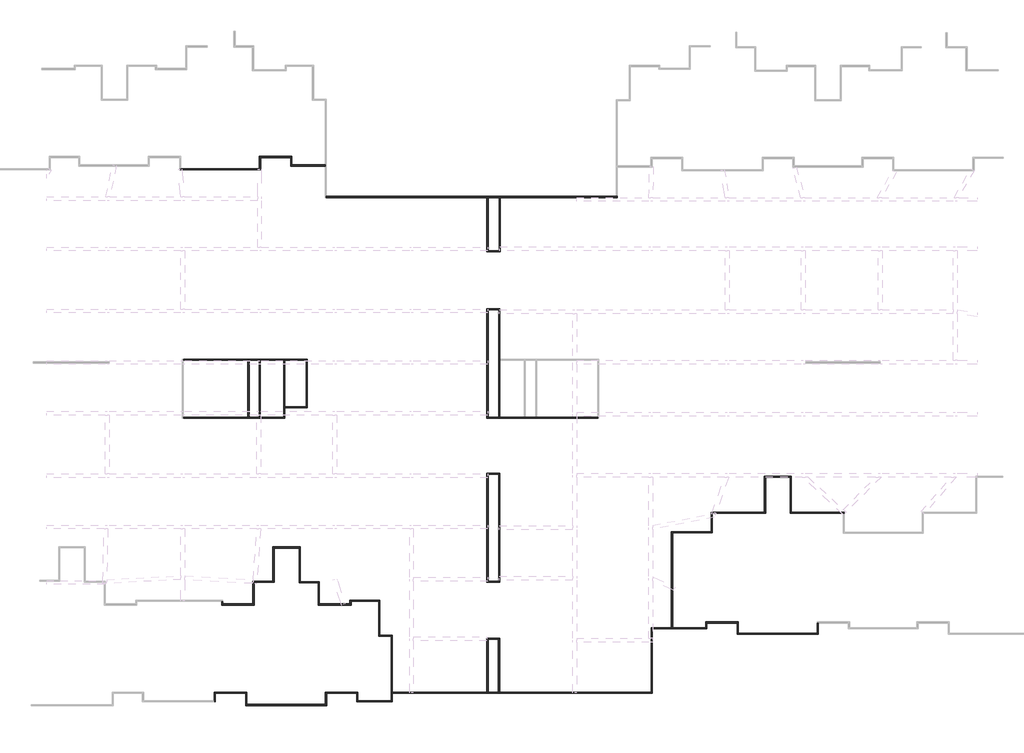
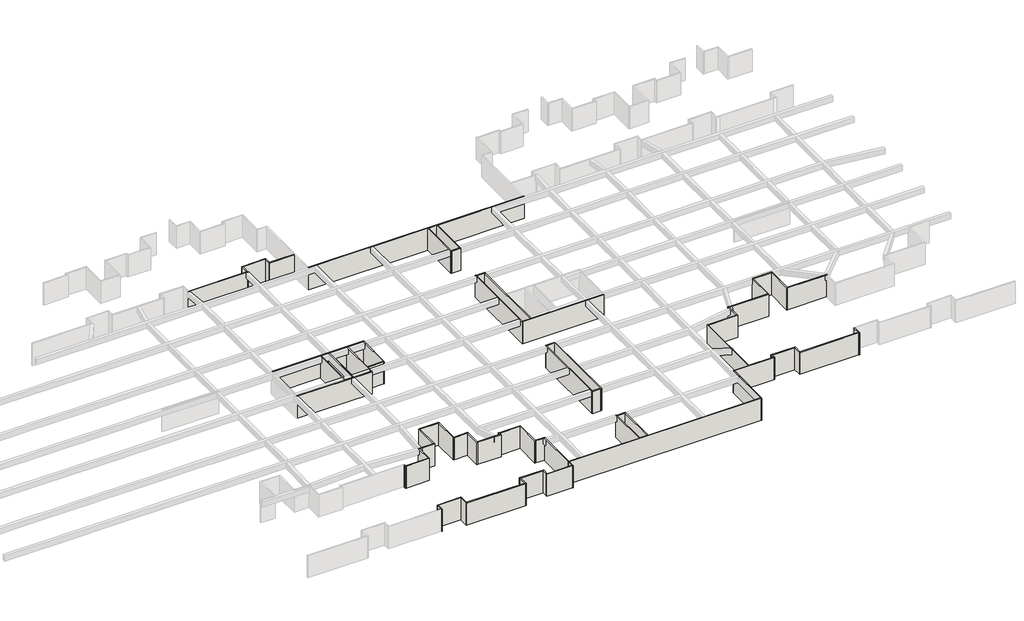
# One storey, part 6 of 16: 67 walls.
"""IFC4 building model written with IfcOpenShell, lengths in millimetres."""

from ifc_helpers import new_model, si_unit, origin, origin_with_axes, place, context, project, spatial, polyline, outline, extrude, faceted_brep, element, save

model = new_model("IFC4")

# Units and contexts
model_context = context("Model", 3, world=origin())
ifc_project = project(units=[si_unit("LENGTHUNIT", "METRE", prefix="MILLI")], contexts=[model_context])

# Site, building, storey
site = spatial("IfcSite", under=ifc_project)
building = spatial("IfcBuilding", under=site)
storey = spatial("IfcBuildingStorey", under=building, Name="户型图", Elevation=0.0)

# Walls
placement = place(None, origin())
element("IfcWall", 1, ObjectType="所有墙体", at=placement, inside=storey, context=model_context, shape_type="Brep", body=[
    faceted_brep([(396205.7298502, -128941.8026441, 0.0), (392717.9162298, -128941.8026441, 0.0), (392597.9162298, -128941.8026441, 0.0), (392597.9162298, -128941.8026441, 3300.0), (392717.9162298, -128941.8026441, 3300.0), (396205.7298502, -128941.8026441, 3300.0), (396205.7298502, -129061.8026441, 0.0), (396205.7298502, -129061.8026441, 3300.0), (392597.9162298, -129061.8026441, 3300.0), (392597.9162298, -129061.8026441, 0.0)], [[[0, 1, 2, 3, 4, 5]], [[6, 7, 8, 9]], [[2, 1, 0, 6, 9]], [[5, 4, 3, 8, 7]], [[0, 5, 7, 6]], [[3, 2, 9, 8]]]),
])
element("IfcWall", 2, ObjectType="所有墙体", at=placement, inside=storey, context=model_context, shape_type="Brep", body=[
    faceted_brep([(392717.9162298, -128941.8026441, 0.0), (392717.9162298, -128039.1416737, 0.0), (392717.9162298, -128039.1416737, 3300.0), (392717.9162298, -128941.8026441, 3300.0), (392597.9162298, -128941.8026441, 0.0), (392597.9162298, -128941.8026441, 3300.0), (392597.9162298, -128159.1416737, 3300.0), (392597.9162298, -128039.1416737, 3300.0), (392597.9162298, -128039.1416737, 0.0), (392597.9162298, -128159.1416737, 0.0)], [[[0, 1, 2, 3]], [[4, 5, 6, 7, 8, 9]], [[1, 0, 4, 9, 8]], [[3, 2, 7, 6, 5]], [[0, 3, 5, 4]], [[2, 1, 8, 7]]]),
])
element("IfcWall", 3, ObjectType="所有墙体", at=placement, inside=storey, context=model_context, shape_type="Brep", body=[
    faceted_brep([(392597.9162298, -128039.1416737, 0.0), (389297.1677555, -128039.1416737, 0.0), (389297.1677555, -128039.1416737, 3300.0), (392597.9162298, -128039.1416737, 3300.0), (392597.9162298, -128159.1416737, 0.0), (392597.9162298, -128159.1416737, 3300.0), (389417.1677555, -128159.1416737, 3300.0), (389297.1677555, -128159.1416737, 3300.0), (389297.1677555, -128159.1416737, 0.0), (389417.1677555, -128159.1416737, 0.0)], [[[0, 1, 2, 3]], [[4, 5, 6, 7, 8, 9]], [[1, 0, 4, 9, 8]], [[3, 2, 7, 6, 5]], [[0, 3, 5, 4]], [[2, 1, 8, 7]]]),
])
element("IfcWall", 4, ObjectType="所有墙体", at=placement, inside=storey, context=model_context, shape_type="Brep", body=[
    faceted_brep([(389297.1677555, -128159.1416737, 0.0), (389297.1677555, -129335.4591871, 0.0), (389297.1677555, -129455.4591871, 0.0), (389297.1677555, -129455.4591871, 3300.0), (389297.1677555, -129335.4591871, 3300.0), (389297.1677555, -128159.1416737, 3300.0), (389417.1677555, -128159.1416737, 0.0), (389417.1677555, -128159.1416737, 3300.0), (389417.1677555, -129455.4591871, 3300.0), (389417.1677555, -129455.4591871, 0.0)], [[[0, 1, 2, 3, 4, 5]], [[6, 7, 8, 9]], [[2, 1, 0, 6, 9]], [[5, 4, 3, 8, 7]], [[0, 5, 7, 6]], [[3, 2, 9, 8]]]),
])
element("IfcWall", 5, ObjectType="所有墙体", at=placement, inside=storey, context=model_context, shape_type="Brep", body=[
    faceted_brep([(389297.1677555, -129335.4591871, 0.0), (381017.0370116, -129335.4591871, 0.0), (380897.0370116, -129335.4591871, 0.0), (380897.0370116, -129335.4591871, 3300.0), (381017.0370116, -129335.4591871, 3300.0), (389297.1677555, -129335.4591871, 3300.0), (389297.1677555, -129455.4591871, 0.0), (389297.1677555, -129455.4591871, 3300.0), (380897.0370116, -129455.4591871, 3300.0), (380897.0370116, -129455.4591871, 0.0)], [[[0, 1, 2, 3, 4, 5]], [[6, 7, 8, 9]], [[2, 1, 0, 6, 9]], [[5, 4, 3, 8, 7]], [[0, 5, 7, 6]], [[3, 2, 9, 8]]]),
])
element("IfcWall", 6, ObjectType="所有墙体", at=placement, inside=storey, context=model_context, shape_type="Brep", body=[
    faceted_brep([(396325.7298502, -132365.1471775, 0.0), (413218.7576761, -132365.1471775, 0.0), (413338.7576761, -132365.1471775, 0.0), (414493.7576761, -132365.1471775, 0.0), (414613.7576761, -132365.1471775, 0.0), (426925.7298502, -132365.1471775, 0.0), (426925.7298502, -132365.1471775, 3300.0), (414613.7576761, -132365.1471775, 3300.0), (414493.7576761, -132365.1471775, 3300.0), (413338.7576761, -132365.1471775, 3300.0), (413218.7576761, -132365.1471775, 3300.0), (396325.7298502, -132365.1471775, 3300.0), (396325.7298502, -132245.1471775, 0.0), (396325.7298502, -132245.1471775, 3300.0), (426805.7298502, -132245.1471775, 3300.0), (426925.7298502, -132245.1471775, 3300.0), (426925.7298502, -132245.1471775, 0.0), (426805.7298502, -132245.1471775, 0.0)], [[[0, 1, 2, 3, 4, 5, 6, 7, 8, 9, 10, 11]], [[12, 13, 14, 15, 16, 17]], [[5, 4, 3, 2, 1, 0, 12, 17, 16]], [[11, 10, 9, 8, 7, 6, 15, 14, 13]], [[0, 11, 13, 12]], [[6, 5, 16, 15]]]),
])
element("IfcWall", 7, ObjectType="所有墙体", at=placement, inside=storey, context=model_context, shape_type="Brep", body=[
    faceted_brep([(447910.2277458, -177096.9317024, 0.0), (447910.2277458, -178176.9317024, 0.0), (447910.2277458, -178296.9317024, 0.0), (447910.2277458, -178296.9317024, 3300.0), (447910.2277458, -178176.9317024, 3300.0), (447910.2277458, -177096.9317024, 3300.0), (448030.2277458, -177096.9317024, 0.0), (448030.2277458, -177096.9317024, 3300.0), (448030.2277458, -178296.9317024, 3300.0), (448030.2277458, -178296.9317024, 0.0)], [[[0, 1, 2, 3, 4, 5]], [[6, 7, 8, 9]], [[2, 1, 0, 6, 9]], [[5, 4, 3, 8, 7]], [[0, 5, 7, 6]], [[3, 2, 9, 8]]]),
])
element("IfcWall", 8, ObjectType="所有墙体", at=placement, inside=storey, context=model_context, shape_type="Brep", body=[
    faceted_brep([(447910.2277458, -178176.9317024, 0.0), (439630.1550834, -178176.9317024, 0.0), (439510.1550834, -178176.9317024, 0.0), (439510.1550834, -178176.9317024, 3300.0), (439630.1550834, -178176.9317024, 3300.0), (447910.2277458, -178176.9317024, 3300.0), (447910.2277458, -178296.9317024, 0.0), (447910.2277458, -178296.9317024, 3300.0), (439510.1550834, -178296.9317024, 3300.0), (439510.1550834, -178296.9317024, 0.0)], [[[0, 1, 2, 3, 4, 5]], [[6, 7, 8, 9]], [[2, 1, 0, 6, 9]], [[5, 4, 3, 8, 7]], [[0, 5, 7, 6]], [[3, 2, 9, 8]]]),
])
element("IfcWall", 9, ObjectType="所有墙体", at=placement, inside=storey, context=model_context, shape_type="Brep", body=[
    faceted_brep([(439630.1550834, -178176.9317024, 0.0), (439630.1550834, -176976.9317024, 0.0), (439630.1550834, -176976.9317024, 3300.0), (439630.1550834, -178176.9317024, 3300.0), (439510.1550834, -178176.9317024, 0.0), (439510.1550834, -178176.9317024, 3300.0), (439510.1550834, -177096.9317024, 3300.0), (439510.1550834, -176976.9317024, 3300.0), (439510.1550834, -176976.9317024, 0.0), (439510.1550834, -177096.9317024, 0.0)], [[[0, 1, 2, 3]], [[4, 5, 6, 7, 8, 9]], [[1, 0, 4, 9, 8]], [[3, 2, 7, 6, 5]], [[0, 3, 5, 4]], [[2, 1, 8, 7]]]),
])
element("IfcWall", 10, ObjectType="所有墙体", at=placement, inside=storey, context=model_context, shape_type="Brep", body=[
    faceted_brep([(439510.1550834, -176976.9317024, 0.0), (436210.2204612, -176976.9317024, 0.0), (436210.2204612, -176976.9317024, 3300.0), (439510.1550834, -176976.9317024, 3300.0), (439510.1550834, -177096.9317024, 0.0), (439510.1550834, -177096.9317024, 3300.0), (436330.2204612, -177096.9317024, 3300.0), (436210.2204612, -177096.9317024, 3300.0), (436210.2204612, -177096.9317024, 0.0), (436330.2204612, -177096.9317024, 0.0)], [[[0, 1, 2, 3]], [[4, 5, 6, 7, 8, 9]], [[1, 0, 4, 9, 8]], [[3, 2, 7, 6, 5]], [[0, 3, 5, 4]], [[2, 1, 8, 7]]]),
])
element("IfcWall", 11, ObjectType="所有墙体", at=placement, inside=storey, context=model_context, shape_type="Brep", body=[
    faceted_brep([(436210.2204612, -177096.9317024, 0.0), (436210.2204612, -177576.9317024, 0.0), (436210.2204612, -177696.9317024, 0.0), (436210.2204612, -177696.9317024, 3300.0), (436210.2204612, -177576.9317024, 3300.0), (436210.2204612, -177096.9317024, 3300.0), (436330.2204612, -177096.9317024, 0.0), (436330.2204612, -177096.9317024, 3300.0), (436330.2204612, -177696.9317024, 3300.0), (436330.2204612, -177696.9317024, 0.0)], [[[0, 1, 2, 3, 4, 5]], [[6, 7, 8, 9]], [[2, 1, 0, 6, 9]], [[5, 4, 3, 8, 7]], [[0, 5, 7, 6]], [[3, 2, 9, 8]]]),
])
element("IfcWall", 12, ObjectType="所有墙体", at=placement, inside=storey, context=model_context, shape_type="Brep", body=[
    faceted_brep([(436210.2204612, -177576.9317024, 0.0), (432730.2204612, -177576.9317024, 0.0), (432610.2204612, -177576.9317024, 0.0), (430493.757676, -177576.9317024, 0.0), (430493.757676, -177576.9317024, 3300.0), (432610.2204612, -177576.9317024, 3300.0), (432730.2204612, -177576.9317024, 3300.0), (436210.2204612, -177576.9317024, 3300.0), (436210.2204612, -177696.9317024, 0.0), (436210.2204612, -177696.9317024, 3300.0), (430613.757676, -177696.9317024, 3300.0), (430493.757676, -177696.9317024, 3300.0), (430493.757676, -177696.9317024, 0.0), (430613.757676, -177696.9317024, 0.0)], [[[0, 1, 2, 3, 4, 5, 6, 7]], [[8, 9, 10, 11, 12, 13]], [[3, 2, 1, 0, 8, 13, 12]], [[7, 6, 5, 4, 11, 10, 9]], [[0, 7, 9, 8]], [[4, 3, 12, 11]]]),
])
element("IfcWall", 13, ObjectType="所有墙体", at=placement, inside=storey, context=model_context, shape_type="Brep", body=[
    faceted_brep([(432730.2204612, -177576.9317024, 0.0), (432730.2204612, -167616.9317024, 0.0), (432730.2204612, -167496.9317024, 0.0), (432730.2204612, -167496.9317024, 3300.0), (432730.2204612, -167616.9317024, 3300.0), (432730.2204612, -177576.9317024, 3300.0), (432610.2204612, -177576.9317024, 0.0), (432610.2204612, -177576.9317024, 3300.0), (432610.2204612, -167496.9317024, 3300.0), (432610.2204612, -167496.9317024, 0.0)], [[[0, 1, 2, 3, 4, 5]], [[6, 7, 8, 9]], [[2, 1, 0, 6, 9]], [[5, 4, 3, 8, 7]], [[0, 5, 7, 6]], [[3, 2, 9, 8]]]),
])
element("IfcWall", 14, ObjectType="所有墙体", at=placement, inside=storey, context=model_context, shape_type="Brep", body=[
    faceted_brep([(432730.2204612, -167616.9317024, 0.0), (436890.2204612, -167616.9317024, 0.0), (436890.2204612, -167616.9317024, 3300.0), (432730.2204612, -167616.9317024, 3300.0), (432730.2204612, -167496.9317024, 0.0), (432730.2204612, -167496.9317024, 3300.0), (436770.2204612, -167496.9317024, 3300.0), (436890.2204612, -167496.9317024, 3300.0), (436890.2204612, -167496.9317024, 0.0), (436770.2204612, -167496.9317024, 0.0)], [[[0, 1, 2, 3]], [[4, 5, 6, 7, 8, 9]], [[1, 0, 4, 9, 8]], [[3, 2, 7, 6, 5]], [[0, 3, 5, 4]], [[2, 1, 8, 7]]]),
])
element("IfcWall", 15, ObjectType="所有墙体", at=placement, inside=storey, context=model_context, shape_type="Brep", body=[
    faceted_brep([(436890.2204612, -167496.9317024, 0.0), (436890.2204612, -165556.0833547, 0.0), (436890.2204612, -165436.0833547, 0.0), (436890.2204612, -165436.0833547, 3300.0), (436890.2204612, -165556.0833547, 3300.0), (436890.2204612, -167496.9317024, 3300.0), (436770.2204612, -167496.9317024, 0.0), (436770.2204612, -167496.9317024, 3300.0), (436770.2204612, -165436.0833547, 3300.0), (436770.2204612, -165436.0833547, 0.0)], [[[0, 1, 2, 3, 4, 5]], [[6, 7, 8, 9]], [[2, 1, 0, 6, 9]], [[5, 4, 3, 8, 7]], [[0, 5, 7, 6]], [[3, 2, 9, 8]]]),
])
element("IfcWall", 16, ObjectType="所有墙体", at=placement, inside=storey, context=model_context, shape_type="Brep", body=[
    faceted_brep([(436890.2204612, -165556.0833547, 0.0), (442510.2204612, -165556.0833547, 0.0), (442510.2204612, -165556.0833547, 3300.0), (436890.2204612, -165556.0833547, 3300.0), (436890.2204612, -165436.0833547, 0.0), (436890.2204612, -165436.0833547, 3300.0), (442390.2204612, -165436.0833547, 3300.0), (442510.2204612, -165436.0833547, 3300.0), (442510.2204612, -165436.0833547, 0.0), (442390.2204612, -165436.0833547, 0.0)], [[[0, 1, 2, 3]], [[4, 5, 6, 7, 8, 9]], [[1, 0, 4, 9, 8]], [[3, 2, 7, 6, 5]], [[0, 3, 5, 4]], [[2, 1, 8, 7]]]),
])
element("IfcWall", 17, ObjectType="所有墙体", at=placement, inside=storey, context=model_context, shape_type="Brep", body=[
    faceted_brep([(442510.2204612, -165436.0833547, 0.0), (442510.2204612, -161762.0157871, 0.0), (442510.2204612, -161642.0157871, 0.0), (442510.2204612, -161642.0157871, 3300.0), (442510.2204612, -161762.0157871, 3300.0), (442510.2204612, -165436.0833547, 3300.0), (442390.2204612, -165436.0833547, 0.0), (442390.2204612, -165436.0833547, 3300.0), (442390.2204612, -161642.0157871, 3300.0), (442390.2204612, -161642.0157871, 0.0)], [[[0, 1, 2, 3, 4, 5]], [[6, 7, 8, 9]], [[2, 1, 0, 6, 9]], [[5, 4, 3, 8, 7]], [[0, 5, 7, 6]], [[3, 2, 9, 8]]]),
])
element("IfcWall", 18, ObjectType="所有墙体", at=placement, inside=storey, context=model_context, shape_type="Brep", body=[
    faceted_brep([(442510.2204612, -161762.0157871, 0.0), (445077.6169744, -161762.0157871, 0.0), (445197.6169744, -161762.0157871, 0.0), (445197.6169744, -161762.0157871, 3300.0), (445077.6169744, -161762.0157871, 3300.0), (442510.2204612, -161762.0157871, 3300.0), (442510.2204612, -161642.0157871, 0.0), (442510.2204612, -161642.0157871, 3300.0), (445197.6169744, -161642.0157871, 3300.0), (445197.6169744, -161642.0157871, 0.0)], [[[0, 1, 2, 3, 4, 5]], [[6, 7, 8, 9]], [[2, 1, 0, 6, 9]], [[5, 4, 3, 8, 7]], [[0, 5, 7, 6]], [[3, 2, 9, 8]]]),
])
element("IfcWall", 19, ObjectType="所有墙体", at=placement, inside=storey, context=model_context, shape_type="Brep", body=[
    faceted_brep([(445077.6169744, -161762.0157871, 0.0), (445077.6169744, -165556.0833547, 0.0), (445077.6169744, -165556.0833547, 3300.0), (445077.6169744, -161762.0157871, 3300.0), (445197.6169744, -161762.0157871, 0.0), (445197.6169744, -161762.0157871, 3300.0), (445197.6169744, -165436.0833547, 3300.0), (445197.6169744, -165556.0833547, 3300.0), (445197.6169744, -165556.0833547, 0.0), (445197.6169744, -165436.0833547, 0.0)], [[[0, 1, 2, 3]], [[4, 5, 6, 7, 8, 9]], [[1, 0, 4, 9, 8]], [[3, 2, 7, 6, 5]], [[0, 3, 5, 4]], [[2, 1, 8, 7]]]),
])
element("IfcWall", 20, ObjectType="所有墙体", at=placement, inside=storey, context=model_context, shape_type="Brep", body=[
    faceted_brep([(445197.6169744, -165556.0833547, 0.0), (450677.6169744, -165556.0833547, 0.0), (450797.6169744, -165556.0833547, 0.0), (450797.6169744, -165556.0833547, 3300.0), (450677.6169744, -165556.0833547, 3300.0), (445197.6169744, -165556.0833547, 3300.0), (445197.6169744, -165436.0833547, 0.0), (445197.6169744, -165436.0833547, 3300.0), (450797.6169744, -165436.0833547, 3300.0), (450797.6169744, -165436.0833547, 0.0)], [[[0, 1, 2, 3, 4, 5]], [[6, 7, 8, 9]], [[2, 1, 0, 6, 9]], [[5, 4, 3, 8, 7]], [[0, 5, 7, 6]], [[3, 2, 9, 8]]]),
])
element("IfcWall", 21, ObjectType="所有墙体", at=placement, inside=storey, context=model_context, shape_type="Brep", body=[
    faceted_brep([(430493.757676, -177696.9317024, 0.0), (430493.757676, -184345.1471774, 0.0), (430493.757676, -184465.1471774, 0.0), (430493.757676, -184465.1471774, 3300.0), (430493.757676, -184345.1471774, 3300.0), (430493.757676, -177696.9317024, 3300.0), (430613.757676, -177696.9317024, 0.0), (430613.757676, -177696.9317024, 3300.0), (430613.757676, -184465.1471774, 3300.0), (430613.757676, -184465.1471774, 0.0)], [[[0, 1, 2, 3, 4, 5]], [[6, 7, 8, 9]], [[2, 1, 0, 6, 9]], [[5, 4, 3, 8, 7]], [[0, 5, 7, 6]], [[3, 2, 9, 8]]]),
])
element("IfcWall", 22, ObjectType="所有墙体", at=placement, inside=storey, context=model_context, shape_type="Brep", body=[
    faceted_brep([(430493.757676, -184345.1471774, 0.0), (414538.7576761, -184345.1471774, 0.0), (414418.7576761, -184345.1471774, 0.0), (413338.7576761, -184345.1471774, 0.0), (413218.7576761, -184345.1471774, 0.0), (403274.1485153, -184345.1471774, 0.0), (403154.1485153, -184345.1471774, 0.0), (403139.3328753, -184345.1471774, 0.0), (403139.3328753, -184345.1471774, 3300.0), (403154.1485153, -184345.1471774, 3300.0), (403274.1485153, -184345.1471774, 3300.0), (413218.7576761, -184345.1471774, 3300.0), (413338.7576761, -184345.1471774, 3300.0), (414418.7576761, -184345.1471774, 3300.0), (414538.7576761, -184345.1471774, 3300.0), (430493.757676, -184345.1471774, 3300.0), (430493.757676, -184465.1471774, 0.0), (430493.757676, -184465.1471774, 3300.0), (403259.3328753, -184465.1471774, 3300.0), (403139.3328753, -184465.1471774, 3300.0), (403139.3328753, -184465.1471774, 0.0), (403259.3328753, -184465.1471774, 0.0)], [[[0, 1, 2, 3, 4, 5, 6, 7, 8, 9, 10, 11, 12, 13, 14, 15]], [[16, 17, 18, 19, 20, 21]], [[7, 6, 5, 4, 3, 2, 1, 0, 16, 21, 20]], [[15, 14, 13, 12, 11, 10, 9, 8, 19, 18, 17]], [[0, 15, 17, 16]], [[8, 7, 20, 19]]]),
])
element("IfcWall", 23, ObjectType="所有墙体", at=placement, inside=storey, context=model_context, shape_type="Brep", body=[
    faceted_brep([(403139.3328753, -184465.1471774, 0.0), (403139.3328753, -185270.5257617, 0.0), (403139.3328753, -185390.5257617, 0.0), (403139.3328753, -185390.5257617, 3300.0), (403139.3328753, -185270.5257617, 3300.0), (403139.3328753, -184465.1471774, 3300.0), (403259.3328753, -184465.1471774, 0.0), (403259.3328753, -184465.1471774, 3300.0), (403259.3328753, -185390.5257617, 3300.0), (403259.3328753, -185390.5257617, 0.0)], [[[0, 1, 2, 3, 4, 5]], [[6, 7, 8, 9]], [[2, 1, 0, 6, 9]], [[5, 4, 3, 8, 7]], [[0, 5, 7, 6]], [[3, 2, 9, 8]]]),
])
element("IfcWall", 24, ObjectType="所有墙体", at=placement, inside=storey, context=model_context, shape_type="Brep", body=[
    faceted_brep([(403139.3328753, -185270.5257617, 0.0), (399656.6728051, -185270.5257617, 0.0), (399536.6728051, -185270.5257617, 0.0), (399536.6728051, -185270.5257617, 3300.0), (399656.6728051, -185270.5257617, 3300.0), (403139.3328753, -185270.5257617, 3300.0), (403139.3328753, -185390.5257617, 0.0), (403139.3328753, -185390.5257617, 3300.0), (399536.6728051, -185390.5257617, 3300.0), (399536.6728051, -185390.5257617, 0.0)], [[[0, 1, 2, 3, 4, 5]], [[6, 7, 8, 9]], [[2, 1, 0, 6, 9]], [[5, 4, 3, 8, 7]], [[0, 5, 7, 6]], [[3, 2, 9, 8]]]),
])
element("IfcWall", 25, ObjectType="所有墙体", at=placement, inside=storey, context=model_context, shape_type="Brep", body=[
    faceted_brep([(399656.6728051, -185270.5257617, 0.0), (399656.6728051, -184345.1471774, 0.0), (399656.6728051, -184345.1471774, 3300.0), (399656.6728051, -185270.5257617, 3300.0), (399536.6728051, -185270.5257617, 0.0), (399536.6728051, -185270.5257617, 3300.0), (399536.6728051, -184465.1471774, 3300.0), (399536.6728051, -184345.1471774, 3300.0), (399536.6728051, -184345.1471774, 0.0), (399536.6728051, -184465.1471774, 0.0)], [[[0, 1, 2, 3]], [[4, 5, 6, 7, 8, 9]], [[1, 0, 4, 9, 8]], [[3, 2, 7, 6, 5]], [[0, 3, 5, 4]], [[2, 1, 8, 7]]]),
])
element("IfcWall", 26, ObjectType="所有墙体", at=placement, inside=storey, context=model_context, shape_type="Brep", body=[
    faceted_brep([(399536.6728051, -184345.1471774, 0.0), (396239.0032896, -184345.1471774, 0.0), (396239.0032896, -184345.1471774, 3300.0), (399536.6728051, -184345.1471774, 3300.0), (399536.6728051, -184465.1471774, 0.0), (399536.6728051, -184465.1471774, 3300.0), (396359.0032896, -184465.1471774, 3300.0), (396239.0032896, -184465.1471774, 3300.0), (396239.0032896, -184465.1471774, 0.0), (396359.0032896, -184465.1471774, 0.0)], [[[0, 1, 2, 3]], [[4, 5, 6, 7, 8, 9]], [[1, 0, 4, 9, 8]], [[3, 2, 7, 6, 5]], [[0, 3, 5, 4]], [[2, 1, 8, 7]]]),
])
element("IfcWall", 27, ObjectType="所有墙体", at=placement, inside=storey, context=model_context, shape_type="Brep", body=[
    faceted_brep([(396239.0032896, -184465.1471774, 0.0), (396239.0032896, -185653.0704256, 0.0), (396239.0032896, -185773.0704256, 0.0), (396239.0032896, -185773.0704256, 3300.0), (396239.0032896, -185653.0704256, 3300.0), (396239.0032896, -184465.1471774, 3300.0), (396359.0032896, -184465.1471774, 0.0), (396359.0032896, -184465.1471774, 3300.0), (396359.0032896, -185773.0704256, 3300.0), (396359.0032896, -185773.0704256, 0.0)], [[[0, 1, 2, 3, 4, 5]], [[6, 7, 8, 9]], [[2, 1, 0, 6, 9]], [[5, 4, 3, 8, 7]], [[0, 5, 7, 6]], [[3, 2, 9, 8]]]),
])
element("IfcWall", 28, ObjectType="所有墙体", at=placement, inside=storey, context=model_context, shape_type="Brep", body=[
    faceted_brep([(396239.0032896, -185653.0704256, 0.0), (387955.6675946, -185653.0704256, 0.0), (387835.6675946, -185653.0704256, 0.0), (387835.6675946, -185653.0704256, 3300.0), (387955.6675946, -185653.0704256, 3300.0), (396239.0032896, -185653.0704256, 3300.0), (396239.0032896, -185773.0704256, 0.0), (396239.0032896, -185773.0704256, 3300.0), (387835.6675946, -185773.0704256, 3300.0), (387835.6675946, -185773.0704256, 0.0)], [[[0, 1, 2, 3, 4, 5]], [[6, 7, 8, 9]], [[2, 1, 0, 6, 9]], [[5, 4, 3, 8, 7]], [[0, 5, 7, 6]], [[3, 2, 9, 8]]]),
])
element("IfcWall", 29, ObjectType="所有墙体", at=placement, inside=storey, context=model_context, shape_type="Brep", body=[
    faceted_brep([(387955.6675946, -185653.0704256, 0.0), (387955.6675946, -184345.1471774, 0.0), (387955.6675946, -184345.1471774, 3300.0), (387955.6675946, -185653.0704256, 3300.0), (387835.6675946, -185653.0704256, 0.0), (387835.6675946, -185653.0704256, 3300.0), (387835.6675946, -184465.1471774, 3300.0), (387835.6675946, -184345.1471774, 3300.0), (387835.6675946, -184345.1471774, 0.0), (387835.6675946, -184465.1471774, 0.0)], [[[0, 1, 2, 3]], [[4, 5, 6, 7, 8, 9]], [[1, 0, 4, 9, 8]], [[3, 2, 7, 6, 5]], [[0, 3, 5, 4]], [[2, 1, 8, 7]]]),
])
element("IfcWall", 30, ObjectType="所有墙体", at=placement, inside=storey, context=model_context, shape_type="Brep", body=[
    faceted_brep([(387835.6675946, -184345.1471774, 0.0), (384538.9658496, -184345.1471774, 0.0), (384538.9658496, -184345.1471774, 3300.0), (387835.6675946, -184345.1471774, 3300.0), (387835.6675946, -184465.1471774, 0.0), (387835.6675946, -184465.1471774, 3300.0), (384658.9658496, -184465.1471774, 3300.0), (384538.9658496, -184465.1471774, 3300.0), (384538.9658496, -184465.1471774, 0.0), (384658.9658496, -184465.1471774, 0.0)], [[[0, 1, 2, 3]], [[4, 5, 6, 7, 8, 9]], [[1, 0, 4, 9, 8]], [[3, 2, 7, 6, 5]], [[0, 3, 5, 4]], [[2, 1, 8, 7]]]),
])
element("IfcWall", 31, ObjectType="所有墙体", at=placement, inside=storey, context=model_context, shape_type="Brep", body=[
    faceted_brep([(384538.9658496, -184465.1471774, 0.0), (384538.9658496, -185270.5257617, 0.0), (384538.9658496, -185390.5257617, 0.0), (384538.9658496, -185390.5257617, 3300.0), (384538.9658496, -185270.5257617, 3300.0), (384538.9658496, -184465.1471774, 3300.0), (384658.9658496, -184465.1471774, 0.0), (384658.9658496, -184465.1471774, 3300.0), (384658.9658496, -185390.5257617, 3300.0), (384658.9658496, -185390.5257617, 0.0)], [[[0, 1, 2, 3, 4, 5]], [[6, 7, 8, 9]], [[2, 1, 0, 6, 9]], [[5, 4, 3, 8, 7]], [[0, 5, 7, 6]], [[3, 2, 9, 8]]]),
])
element("IfcWall", 32, ObjectType="所有墙体", at=placement, inside=storey, context=model_context, shape_type="Brep", body=[
    faceted_brep([(385313.3623471, -174822.5388289, 0.0), (385313.3623471, -175202.0297951, 0.0), (385313.3623471, -175202.0297951, 3300.0), (385313.3623471, -174822.5388289, 3300.0), (385433.3623471, -174822.5388289, 0.0), (385433.3623471, -174822.5388289, 3300.0), (385433.3623471, -175082.0297951, 3300.0), (385433.3623471, -175202.0297951, 3300.0), (385433.3623471, -175202.0297951, 0.0), (385433.3623471, -175082.0297951, 0.0)], [[[0, 1, 2, 3]], [[4, 5, 6, 7, 8, 9]], [[1, 0, 4, 9, 8]], [[3, 2, 7, 6, 5]], [[0, 3, 5, 4]], [[2, 1, 8, 7]]]),
])
element("IfcWall", 33, ObjectType="所有墙体", at=placement, inside=storey, context=model_context, shape_type="Brep", body=[
    faceted_brep([(385433.3623471, -175202.0297951, 0.0), (388732.4128619, -175202.0297951, 0.0), (388732.4128619, -175202.0297951, 3300.0), (385433.3623471, -175202.0297951, 3300.0), (385433.3623471, -175082.0297951, 0.0), (385433.3623471, -175082.0297951, 3300.0), (388612.4128619, -175082.0297951, 3300.0), (388732.4128619, -175082.0297951, 3300.0), (388732.4128619, -175082.0297951, 0.0), (388612.4128619, -175082.0297951, 0.0)], [[[0, 1, 2, 3]], [[4, 5, 6, 7, 8, 9]], [[1, 0, 4, 9, 8]], [[3, 2, 7, 6, 5]], [[0, 3, 5, 4]], [[2, 1, 8, 7]]]),
])
element("IfcWall", 34, ObjectType="所有墙体", at=placement, inside=storey, context=model_context, shape_type="Brep", body=[
    faceted_brep([(388732.4128619, -175082.0297951, 0.0), (388732.4128619, -172802.0297951, 0.0), (388732.4128619, -172682.0297951, 0.0), (388732.4128619, -172682.0297951, 3300.0), (388732.4128619, -172802.0297951, 3300.0), (388732.4128619, -175082.0297951, 3300.0), (388612.4128619, -175082.0297951, 0.0), (388612.4128619, -175082.0297951, 3300.0), (388612.4128619, -172682.0297951, 3300.0), (388612.4128619, -172682.0297951, 0.0)], [[[0, 1, 2, 3, 4, 5]], [[6, 7, 8, 9]], [[2, 1, 0, 6, 9]], [[5, 4, 3, 8, 7]], [[0, 5, 7, 6]], [[3, 2, 9, 8]]]),
])
element("IfcWall", 35, ObjectType="所有墙体", at=placement, inside=storey, context=model_context, shape_type="Brep", body=[
    faceted_brep([(388732.4128619, -172802.0297951, 0.0), (390838.4911583, -172802.0297951, 0.0), (390838.4911583, -172802.0297951, 3300.0), (388732.4128619, -172802.0297951, 3300.0), (388732.4128619, -172682.0297951, 0.0), (388732.4128619, -172682.0297951, 3300.0), (390718.4911583, -172682.0297951, 3300.0), (390838.4911583, -172682.0297951, 3300.0), (390838.4911583, -172682.0297951, 0.0), (390718.4911583, -172682.0297951, 0.0)], [[[0, 1, 2, 3]], [[4, 5, 6, 7, 8, 9]], [[1, 0, 4, 9, 8]], [[3, 2, 7, 6, 5]], [[0, 3, 5, 4]], [[2, 1, 8, 7]]]),
])
element("IfcWall", 36, ObjectType="所有墙体", at=placement, inside=storey, context=model_context, shape_type="Brep", body=[
    faceted_brep([(390838.4911583, -172682.0297951, 0.0), (390838.4911583, -169209.0515441, 0.0), (390838.4911583, -169089.0515441, 0.0), (390838.4911583, -169089.0515441, 3300.0), (390838.4911583, -169209.0515441, 3300.0), (390838.4911583, -172682.0297951, 3300.0), (390718.4911583, -172682.0297951, 0.0), (390718.4911583, -172682.0297951, 3300.0), (390718.4911583, -169089.0515441, 3300.0), (390718.4911583, -169089.0515441, 0.0)], [[[0, 1, 2, 3, 4, 5]], [[6, 7, 8, 9]], [[2, 1, 0, 6, 9]], [[5, 4, 3, 8, 7]], [[0, 5, 7, 6]], [[3, 2, 9, 8]]]),
])
element("IfcWall", 37, ObjectType="所有墙体", at=placement, inside=storey, context=model_context, shape_type="Brep", body=[
    faceted_brep([(390838.4911583, -169209.0515441, 0.0), (393477.5895592, -169209.0515441, 0.0), (393597.5895592, -169209.0515441, 0.0), (393597.5895592, -169209.0515441, 3300.0), (393477.5895592, -169209.0515441, 3300.0), (390838.4911583, -169209.0515441, 3300.0), (390838.4911583, -169089.0515441, 0.0), (390838.4911583, -169089.0515441, 3300.0), (393597.5895592, -169089.0515441, 3300.0), (393597.5895592, -169089.0515441, 0.0)], [[[0, 1, 2, 3, 4, 5]], [[6, 7, 8, 9]], [[2, 1, 0, 6, 9]], [[5, 4, 3, 8, 7]], [[0, 5, 7, 6]], [[3, 2, 9, 8]]]),
])
element("IfcWall", 38, ObjectType="所有墙体", at=placement, inside=storey, context=model_context, shape_type="Brep", body=[
    faceted_brep([(393477.5895592, -169209.0515441, 0.0), (393477.5895592, -172866.0432562, 0.0), (393477.5895592, -172866.0432562, 3300.0), (393477.5895592, -169209.0515441, 3300.0), (393597.5895592, -169209.0515441, 0.0), (393597.5895592, -169209.0515441, 3300.0), (393597.5895592, -172746.0432562, 3300.0), (393597.5895592, -172866.0432562, 3300.0), (393597.5895592, -172866.0432562, 0.0), (393597.5895592, -172746.0432562, 0.0)], [[[0, 1, 2, 3]], [[4, 5, 6, 7, 8, 9]], [[1, 0, 4, 9, 8]], [[3, 2, 7, 6, 5]], [[0, 3, 5, 4]], [[2, 1, 8, 7]]]),
])
element("IfcWall", 39, ObjectType="所有墙体", at=placement, inside=storey, context=model_context, shape_type="Brep", body=[
    faceted_brep([(393597.5895592, -172866.0432562, 0.0), (395477.5895592, -172866.0432562, 0.0), (395597.5895592, -172866.0432562, 0.0), (395597.5895592, -172866.0432562, 3300.0), (395477.5895592, -172866.0432562, 3300.0), (393597.5895592, -172866.0432562, 3300.0), (393597.5895592, -172746.0432562, 0.0), (393597.5895592, -172746.0432562, 3300.0), (395597.5895592, -172746.0432562, 3300.0), (395597.5895592, -172746.0432562, 0.0)], [[[0, 1, 2, 3, 4, 5]], [[6, 7, 8, 9]], [[2, 1, 0, 6, 9]], [[5, 4, 3, 8, 7]], [[0, 5, 7, 6]], [[3, 2, 9, 8]]]),
])
element("IfcWall", 40, ObjectType="所有墙体", at=placement, inside=storey, context=model_context, shape_type="Brep", body=[
    faceted_brep([(395477.5895592, -172866.0432562, 0.0), (395477.5895592, -175202.0297951, 0.0), (395477.5895592, -175202.0297951, 3300.0), (395477.5895592, -172866.0432562, 3300.0), (395597.5895592, -172866.0432562, 0.0), (395597.5895592, -172866.0432562, 3300.0), (395597.5895592, -175082.0297951, 3300.0), (395597.5895592, -175202.0297951, 3300.0), (395597.5895592, -175202.0297951, 0.0), (395597.5895592, -175082.0297951, 0.0)], [[[0, 1, 2, 3]], [[4, 5, 6, 7, 8, 9]], [[1, 0, 4, 9, 8]], [[3, 2, 7, 6, 5]], [[0, 3, 5, 4]], [[2, 1, 8, 7]]]),
])
element("IfcWall", 41, ObjectType="所有墙体", at=placement, inside=storey, context=model_context, shape_type="Brep", body=[
    faceted_brep([(395597.5895592, -175202.0297951, 0.0), (398932.4455019, -175202.0297951, 0.0), (398932.4455019, -175202.0297951, 3300.0), (395597.5895592, -175202.0297951, 3300.0), (395597.5895592, -175082.0297951, 0.0), (395597.5895592, -175082.0297951, 3300.0), (398812.4455019, -175082.0297951, 3300.0), (398932.4455019, -175082.0297951, 3300.0), (398932.4455019, -175082.0297951, 0.0), (398812.4455019, -175082.0297951, 0.0)], [[[0, 1, 2, 3]], [[4, 5, 6, 7, 8, 9]], [[1, 0, 4, 9, 8]], [[3, 2, 7, 6, 5]], [[0, 3, 5, 4]], [[2, 1, 8, 7]]]),
])
element("IfcWall", 42, ObjectType="所有墙体", at=placement, inside=storey, context=model_context, shape_type="Brep", body=[
    faceted_brep([(398932.4455019, -175082.0297951, 0.0), (398932.4455019, -174822.5388289, 0.0), (398932.4455019, -174702.5388289, 0.0), (398932.4455019, -174702.5388289, 3300.0), (398932.4455019, -174822.5388289, 3300.0), (398932.4455019, -175082.0297951, 3300.0), (398812.4455019, -175082.0297951, 0.0), (398812.4455019, -175082.0297951, 3300.0), (398812.4455019, -174702.5388289, 3300.0), (398812.4455019, -174702.5388289, 0.0)], [[[0, 1, 2, 3, 4, 5]], [[6, 7, 8, 9]], [[2, 1, 0, 6, 9]], [[5, 4, 3, 8, 7]], [[0, 5, 7, 6]], [[3, 2, 9, 8]]]),
])
element("IfcWall", 43, ObjectType="所有墙体", at=placement, inside=storey, context=model_context, shape_type="Brep", body=[
    faceted_brep([(398932.4455019, -174822.5388289, 0.0), (401813.4151471, -174822.5388289, 0.0), (401933.4151471, -174822.5388289, 0.0), (401933.4151471, -174822.5388289, 3300.0), (401813.4151471, -174822.5388289, 3300.0), (398932.4455019, -174822.5388289, 3300.0), (398932.4455019, -174702.5388289, 0.0), (398932.4455019, -174702.5388289, 3300.0), (401933.4151471, -174702.5388289, 3300.0), (401933.4151471, -174702.5388289, 0.0)], [[[0, 1, 2, 3, 4, 5]], [[6, 7, 8, 9]], [[2, 1, 0, 6, 9]], [[5, 4, 3, 8, 7]], [[0, 5, 7, 6]], [[3, 2, 9, 8]]]),
])
element("IfcWall", 44, ObjectType="所有墙体", at=placement, inside=storey, context=model_context, shape_type="Brep", body=[
    faceted_brep([(401813.4151471, -174822.5388289, 0.0), (401813.4151471, -178487.2022403, 0.0), (401813.4151471, -178487.2022403, 3300.0), (401813.4151471, -174822.5388289, 3300.0), (401933.4151471, -174822.5388289, 0.0), (401933.4151471, -174822.5388289, 3300.0), (401933.4151471, -178367.2022403, 3300.0), (401933.4151471, -178487.2022403, 3300.0), (401933.4151471, -178487.2022403, 0.0), (401933.4151471, -178367.2022403, 0.0)], [[[0, 1, 2, 3]], [[4, 5, 6, 7, 8, 9]], [[1, 0, 4, 9, 8]], [[3, 2, 7, 6, 5]], [[0, 3, 5, 4]], [[2, 1, 8, 7]]]),
])
element("IfcWall", 45, ObjectType="所有墙体", at=placement, inside=storey, context=model_context, shape_type="Brep", body=[
    faceted_brep([(401933.4151471, -178487.2022403, 0.0), (403154.1485153, -178487.2022403, 0.0), (403274.1485153, -178487.2022403, 0.0), (403274.1485153, -178487.2022403, 3300.0), (403154.1485153, -178487.2022403, 3300.0), (401933.4151471, -178487.2022403, 3300.0), (401933.4151471, -178367.2022403, 0.0), (401933.4151471, -178367.2022403, 3300.0), (403274.1485153, -178367.2022403, 3300.0), (403274.1485153, -178367.2022403, 0.0)], [[[0, 1, 2, 3, 4, 5]], [[6, 7, 8, 9]], [[2, 1, 0, 6, 9]], [[5, 4, 3, 8, 7]], [[0, 5, 7, 6]], [[3, 2, 9, 8]]]),
])
element("IfcWall", 46, ObjectType="所有墙体", at=placement, inside=storey, context=model_context, shape_type="SweptSolid", body=[
    extrude(outline(polyline([(403154.1485153, -184345.1471774), (403154.1485153, -178487.2022403), (403274.1485153, -178487.2022403), (403274.1485153, -184345.1471774), (403154.1485153, -184345.1471774)])), origin_with_axes(), (0.0, 0.0, 1.0), 3300.0),
])
element("IfcWall", 47, ObjectType="所有墙体", at=placement, inside=storey, context=model_context, shape_type="Brep", body=[
    faceted_brep([(413218.7576761, -132365.1471775, 0.0), (413218.7576761, -138065.1471775, 0.0), (413218.7576761, -138065.1471775, 3300.0), (413218.7576761, -132365.1471775, 3300.0), (413338.7576761, -132365.1471775, 0.0), (413338.7576761, -132365.1471775, 3300.0), (413338.7576761, -137945.1471775, 3300.0), (413338.7576761, -138065.1471775, 3300.0), (413338.7576761, -138065.1471775, 0.0), (413338.7576761, -137945.1471775, 0.0)], [[[0, 1, 2, 3]], [[4, 5, 6, 7, 8, 9]], [[1, 0, 4, 9, 8]], [[3, 2, 7, 6, 5]], [[0, 3, 5, 4]], [[2, 1, 8, 7]]]),
])
element("IfcWall", 48, ObjectType="所有墙体", at=placement, inside=storey, context=model_context, shape_type="Brep", body=[
    faceted_brep([(413338.7576761, -138065.1471775, 0.0), (414613.7576761, -138065.1471775, 0.0), (414613.7576761, -138065.1471775, 3300.0), (413338.7576761, -138065.1471775, 3300.0), (413338.7576761, -137945.1471775, 0.0), (413338.7576761, -137945.1471775, 3300.0), (414493.7576761, -137945.1471775, 3300.0), (414613.7576761, -137945.1471775, 3300.0), (414613.7576761, -137945.1471775, 0.0), (414493.7576761, -137945.1471775, 0.0)], [[[0, 1, 2, 3]], [[4, 5, 6, 7, 8, 9]], [[1, 0, 4, 9, 8]], [[3, 2, 7, 6, 5]], [[0, 3, 5, 4]], [[2, 1, 8, 7]]]),
])
element("IfcWall", 49, ObjectType="所有墙体", at=placement, inside=storey, context=model_context, shape_type="SweptSolid", body=[
    extrude(outline(polyline([(414613.7576761, -132365.1471775), (414613.7576761, -137945.1471775), (414493.7576761, -137945.1471775), (414493.7576761, -132365.1471775), (414613.7576761, -132365.1471775)])), origin_with_axes(), (0.0, 0.0, 1.0), 3300.0),
])
element("IfcWall", 50, ObjectType="所有墙体", at=placement, inside=storey, context=model_context, shape_type="Brep", body=[
    faceted_brep([(413218.7576761, -144045.1471774, 0.0), (413218.7576761, -155565.1471774, 0.0), (413218.7576761, -155565.1471774, 3300.0), (413218.7576761, -144045.1471774, 3300.0), (413338.7576761, -144045.1471774, 0.0), (413338.7576761, -144045.1471774, 3300.0), (413338.7576761, -144165.1471774, 3300.0), (413338.7576761, -155445.1471774, 3300.0), (413338.7576761, -155565.1471774, 3300.0), (413338.7576761, -155565.1471774, 0.0), (413338.7576761, -155445.1471774, 0.0), (413338.7576761, -144165.1471774, 0.0)], [[[0, 1, 2, 3]], [[4, 5, 6, 7, 8, 9, 10, 11]], [[1, 0, 4, 11, 10, 9]], [[3, 2, 8, 7, 6, 5]], [[2, 1, 9, 8]], [[0, 3, 5, 4]]]),
])
element("IfcWall", 51, ObjectType="所有墙体", at=placement, inside=storey, context=model_context, shape_type="Brep", body=[
    faceted_brep([(413338.7576761, -155565.1471774, 0.0), (424843.757676, -155565.1471774, 0.0), (424843.757676, -155565.1471774, 3300.0), (413338.7576761, -155565.1471774, 3300.0), (413338.7576761, -155445.1471774, 0.0), (413338.7576761, -155445.1471774, 3300.0), (414443.7576761, -155445.1471774, 3300.0), (414563.7576761, -155445.1471774, 3300.0), (417143.7576761, -155445.1471774, 3300.0), (417263.7576761, -155445.1471774, 3300.0), (418343.7576761, -155445.1471774, 3300.0), (418463.7576761, -155445.1471774, 3300.0), (424843.757676, -155445.1471774, 3300.0), (424843.757676, -155445.1471774, 0.0), (418463.7576761, -155445.1471774, 0.0), (418343.7576761, -155445.1471774, 0.0), (417263.7576761, -155445.1471774, 0.0), (417143.7576761, -155445.1471774, 0.0), (414563.7576761, -155445.1471774, 0.0), (414443.7576761, -155445.1471774, 0.0)], [[[0, 1, 2, 3]], [[4, 5, 6, 7, 8, 9, 10, 11, 12, 13, 14, 15, 16, 17, 18, 19]], [[1, 0, 4, 19, 18, 17, 16, 15, 14, 13]], [[3, 2, 12, 11, 10, 9, 8, 7, 6, 5]], [[0, 3, 5, 4]], [[2, 1, 13, 12]]]),
])
element("IfcWall", 52, ObjectType="所有墙体", at=placement, inside=storey, context=model_context, shape_type="Brep", body=[
    faceted_brep([(414563.7576761, -155445.1471774, 0.0), (414563.7576761, -149465.1471774, 0.0), (414563.7576761, -149345.1471774, 0.0), (414563.7576761, -144045.1471774, 0.0), (414563.7576761, -144045.1471774, 3300.0), (414563.7576761, -149345.1471774, 3300.0), (414563.7576761, -149465.1471774, 3300.0), (414563.7576761, -155445.1471774, 3300.0), (414443.7576761, -155445.1471774, 0.0), (414443.7576761, -155445.1471774, 3300.0), (414443.7576761, -144165.1471774, 3300.0), (414443.7576761, -144045.1471774, 3300.0), (414443.7576761, -144045.1471774, 0.0), (414443.7576761, -144165.1471774, 0.0)], [[[0, 1, 2, 3, 4, 5, 6, 7]], [[8, 9, 10, 11, 12, 13]], [[3, 2, 1, 0, 8, 13, 12]], [[7, 6, 5, 4, 11, 10, 9]], [[0, 7, 9, 8]], [[4, 3, 12, 11]]]),
])
element("IfcWall", 53, ObjectType="所有墙体", at=placement, inside=storey, context=model_context, shape_type="SweptSolid", body=[
    extrude(outline(polyline([(413338.7576761, -144045.1471774), (414443.7576761, -144045.1471774), (414443.7576761, -144165.1471774), (413338.7576761, -144165.1471774), (413338.7576761, -144045.1471774)])), origin_with_axes(), (0.0, 0.0, 1.0), 3300.0),
])
element("IfcWall", 54, ObjectType="所有墙体", at=placement, inside=storey, context=model_context, shape_type="Brep", body=[
    faceted_brep([(413218.7576761, -161462.0157871, 0.0), (413338.7576761, -161462.0157871, 0.0), (414443.7576761, -161462.0157871, 0.0), (414563.7576761, -161462.0157871, 0.0), (414563.7576761, -161462.0157871, 3300.0), (414443.7576761, -161462.0157871, 3300.0), (413338.7576761, -161462.0157871, 3300.0), (413218.7576761, -161462.0157871, 3300.0), (413218.7576761, -161342.0157871, 0.0), (413218.7576761, -161342.0157871, 3300.0), (414563.7576761, -161342.0157871, 3300.0), (414563.7576761, -161342.0157871, 0.0)], [[[0, 1, 2, 3, 4, 5, 6, 7]], [[8, 9, 10, 11]], [[3, 2, 1, 0, 8, 11]], [[7, 6, 5, 4, 10, 9]], [[4, 3, 11, 10]], [[0, 7, 9, 8]]]),
])
element("IfcWall", 55, ObjectType="所有墙体", at=placement, inside=storey, context=model_context, shape_type="Brep", body=[
    faceted_brep([(414443.7576761, -161462.0157871, 0.0), (414443.7576761, -172682.0297951, 0.0), (414443.7576761, -172802.0297951, 0.0), (414443.7576761, -172802.0297951, 3300.0), (414443.7576761, -172682.0297951, 3300.0), (414443.7576761, -161462.0157871, 3300.0), (414563.7576761, -161462.0157871, 0.0), (414563.7576761, -161462.0157871, 3300.0), (414563.7576761, -172802.0297951, 3300.0), (414563.7576761, -172802.0297951, 0.0)], [[[0, 1, 2, 3, 4, 5]], [[6, 7, 8, 9]], [[2, 1, 0, 6, 9]], [[5, 4, 3, 8, 7]], [[0, 5, 7, 6]], [[3, 2, 9, 8]]]),
])
element("IfcWall", 56, ObjectType="所有墙体", at=placement, inside=storey, context=model_context, shape_type="Brep", body=[
    faceted_brep([(414443.7576761, -172682.0297951, 0.0), (413338.7576761, -172682.0297951, 0.0), (413218.7576761, -172682.0297951, 0.0), (413218.7576761, -172682.0297951, 3300.0), (413338.7576761, -172682.0297951, 3300.0), (414443.7576761, -172682.0297951, 3300.0), (414443.7576761, -172802.0297951, 0.0), (414443.7576761, -172802.0297951, 3300.0), (413218.7576761, -172802.0297951, 3300.0), (413218.7576761, -172802.0297951, 0.0)], [[[0, 1, 2, 3, 4, 5]], [[6, 7, 8, 9]], [[2, 1, 0, 6, 9]], [[5, 4, 3, 8, 7]], [[0, 5, 7, 6]], [[3, 2, 9, 8]]]),
])
element("IfcWall", 57, ObjectType="所有墙体", at=placement, inside=storey, context=model_context, shape_type="SweptSolid", body=[
    extrude(outline(polyline([(413338.7576761, -161462.0157871), (413338.7576761, -172682.0297951), (413218.7576761, -172682.0297951), (413218.7576761, -161462.0157871), (413338.7576761, -161462.0157871)])), origin_with_axes(), (0.0, 0.0, 1.0), 3300.0),
])
element("IfcWall", 58, ObjectType="所有墙体", at=placement, inside=storey, context=model_context, shape_type="Brep", body=[
    faceted_brep([(381313.757676, -155565.1471774, 0.0), (391963.757676, -155565.1471774, 0.0), (391963.757676, -155565.1471774, 3300.0), (381313.757676, -155565.1471774, 3300.0), (381313.757676, -155445.1471774, 0.0), (381313.757676, -155445.1471774, 3300.0), (388093.757676, -155445.1471774, 3300.0), (388213.757676, -155445.1471774, 3300.0), (389253.757676, -155445.1471774, 3300.0), (389373.757676, -155445.1471774, 3300.0), (391843.757676, -155445.1471774, 3300.0), (391963.757676, -155445.1471774, 3300.0), (391963.757676, -155445.1471774, 0.0), (391843.757676, -155445.1471774, 0.0), (389373.757676, -155445.1471774, 0.0), (389253.757676, -155445.1471774, 0.0), (388213.757676, -155445.1471774, 0.0), (388093.757676, -155445.1471774, 0.0)], [[[0, 1, 2, 3]], [[4, 5, 6, 7, 8, 9, 10, 11, 12, 13, 14, 15, 16, 17]], [[1, 0, 4, 17, 16, 15, 14, 13, 12]], [[3, 2, 11, 10, 9, 8, 7, 6, 5]], [[0, 3, 5, 4]], [[2, 1, 12, 11]]]),
])
element("IfcWall", 59, ObjectType="所有墙体", at=placement, inside=storey, context=model_context, shape_type="Brep", body=[
    faceted_brep([(391963.757676, -155445.1471774, 0.0), (391963.757676, -154465.1471774, 0.0), (391963.757676, -154345.1471774, 0.0), (391963.757676, -149465.1471774, 0.0), (391963.757676, -149465.1471774, 3300.0), (391963.757676, -154345.1471774, 3300.0), (391963.757676, -154465.1471774, 3300.0), (391963.757676, -155445.1471774, 3300.0), (391843.757676, -155445.1471774, 0.0), (391843.757676, -155445.1471774, 3300.0), (391843.757676, -149465.1471774, 3300.0), (391843.757676, -149465.1471774, 0.0)], [[[0, 1, 2, 3, 4, 5, 6, 7]], [[8, 9, 10, 11]], [[3, 2, 1, 0, 8, 11]], [[7, 6, 5, 4, 10, 9]], [[0, 7, 9, 8]], [[4, 3, 11, 10]]]),
])
element("IfcWall", 60, ObjectType="所有墙体", at=placement, inside=storey, context=model_context, shape_type="Brep", body=[
    faceted_brep([(394313.757676, -149345.1471774, 0.0), (381313.757676, -149345.1471774, 0.0), (381313.757676, -149345.1471774, 3300.0), (394313.757676, -149345.1471774, 3300.0), (394313.757676, -149465.1471774, 0.0), (394313.757676, -149465.1471774, 3300.0), (394193.757676, -149465.1471774, 3300.0), (391963.757676, -149465.1471774, 3300.0), (391843.757676, -149465.1471774, 3300.0), (389373.757676, -149465.1471774, 3300.0), (389253.757676, -149465.1471774, 3300.0), (388213.757676, -149465.1471774, 3300.0), (388093.757676, -149465.1471774, 3300.0), (381313.757676, -149465.1471774, 3300.0), (381313.757676, -149465.1471774, 0.0), (388093.757676, -149465.1471774, 0.0), (388213.757676, -149465.1471774, 0.0), (389253.757676, -149465.1471774, 0.0), (389373.757676, -149465.1471774, 0.0), (391843.757676, -149465.1471774, 0.0), (391963.757676, -149465.1471774, 0.0), (394193.757676, -149465.1471774, 0.0)], [[[0, 1, 2, 3]], [[4, 5, 6, 7, 8, 9, 10, 11, 12, 13, 14, 15, 16, 17, 18, 19, 20, 21]], [[1, 0, 4, 21, 20, 19, 18, 17, 16, 15, 14]], [[3, 2, 13, 12, 11, 10, 9, 8, 7, 6, 5]], [[2, 1, 14, 13]], [[0, 3, 5, 4]]]),
])
element("IfcWall", 61, ObjectType="所有墙体", at=placement, inside=storey, context=model_context, shape_type="SweptSolid", body=[
    extrude(outline(polyline([(388093.757676, -155445.1471774), (388093.757676, -149465.1471774), (388213.757676, -149465.1471774), (388213.757676, -155445.1471774), (388093.757676, -155445.1471774)])), origin_with_axes(), (0.0, 0.0, 1.0), 3300.0),
])
element("IfcWall", 62, ObjectType="所有墙体", at=placement, inside=storey, context=model_context, shape_type="SweptSolid", body=[
    extrude(outline(polyline([(389253.757676, -155445.1471774), (389253.757676, -149465.1471774), (389373.757676, -149465.1471774), (389373.757676, -155445.1471774), (389253.757676, -155445.1471774)])), origin_with_axes(), (0.0, 0.0, 1.0), 3300.0),
])
element("IfcWall", 63, ObjectType="所有墙体", at=placement, inside=storey, context=model_context, shape_type="Brep", body=[
    faceted_brep([(394193.757676, -149465.1471774, 0.0), (394193.757676, -154345.1471774, 0.0), (394193.757676, -154465.1471774, 0.0), (394193.757676, -154465.1471774, 3300.0), (394193.757676, -154345.1471774, 3300.0), (394193.757676, -149465.1471774, 3300.0), (394313.757676, -149465.1471774, 0.0), (394313.757676, -149465.1471774, 3300.0), (394313.757676, -154465.1471774, 3300.0), (394313.757676, -154465.1471774, 0.0)], [[[0, 1, 2, 3, 4, 5]], [[6, 7, 8, 9]], [[2, 1, 0, 6, 9]], [[5, 4, 3, 8, 7]], [[0, 5, 7, 6]], [[3, 2, 9, 8]]]),
])
element("IfcWall", 64, ObjectType="所有墙体", at=placement, inside=storey, context=model_context, shape_type="SweptSolid", body=[
    extrude(outline(polyline([(391963.757676, -154345.1471774), (394193.757676, -154345.1471774), (394193.757676, -154465.1471774), (391963.757676, -154465.1471774), (391963.757676, -154345.1471774)])), origin_with_axes(), (0.0, 0.0, 1.0), 3300.0),
])
element("IfcWall", 65, ObjectType="所有墙体", at=placement, inside=storey, context=model_context, shape_type="Brep", body=[
    faceted_brep([(413338.7576761, -184345.1471774, 0.0), (413338.7576761, -178796.89075, 0.0), (413338.7576761, -178676.89075, 0.0), (413338.7576761, -178676.89075, 3300.0), (413338.7576761, -178796.89075, 3300.0), (413338.7576761, -184345.1471774, 3300.0), (413218.7576761, -184345.1471774, 0.0), (413218.7576761, -184345.1471774, 3300.0), (413218.7576761, -178676.89075, 3300.0), (413218.7576761, -178676.89075, 0.0)], [[[0, 1, 2, 3, 4, 5]], [[6, 7, 8, 9]], [[2, 1, 0, 6, 9]], [[5, 4, 3, 8, 7]], [[0, 5, 7, 6]], [[3, 2, 9, 8]]]),
])
element("IfcWall", 66, ObjectType="所有墙体", at=placement, inside=storey, context=model_context, shape_type="Brep", body=[
    faceted_brep([(413338.7576761, -178796.89075, 0.0), (414418.7576761, -178796.89075, 0.0), (414538.7576761, -178796.89075, 0.0), (414538.7576761, -178796.89075, 3300.0), (414418.7576761, -178796.89075, 3300.0), (413338.7576761, -178796.89075, 3300.0), (413338.7576761, -178676.89075, 0.0), (413338.7576761, -178676.89075, 3300.0), (414538.7576761, -178676.89075, 3300.0), (414538.7576761, -178676.89075, 0.0)], [[[0, 1, 2, 3, 4, 5]], [[6, 7, 8, 9]], [[2, 1, 0, 6, 9]], [[5, 4, 3, 8, 7]], [[0, 5, 7, 6]], [[3, 2, 9, 8]]]),
])
element("IfcWall", 67, ObjectType="所有墙体", at=placement, inside=storey, context=model_context, shape_type="SweptSolid", body=[
    extrude(outline(polyline([(414418.7576761, -184345.1471774), (414418.7576761, -178796.89075), (414538.7576761, -178796.89075), (414538.7576761, -184345.1471774), (414418.7576761, -184345.1471774)])), origin_with_axes(), (0.0, 0.0, 1.0), 3300.0),
])

save(model, "model.ifc")

# Revit data of these elements
# Type "所有墙体"
#   Layers, outside or top first: 120 mm "默认" (function 1)
# Elements 1, 2, 3, 4, 5, 6, 7, 8, 9, 10, 11, 12, 13, 14, 15, 16, 17, 18, 19, 20, 21, 22, 23, 24, 25, 26, 27, 28, 29, 30, 31, 32, 33, 34, 35, 36, 37, 38, 39, 40, 41, 42, 43, 44, 45, 46, 47, 48, 49, 50, 51, 52, 53, 54, 55, 56, 57, 58, 59, 60, 61, 62, 63, 64, 65, 66, 67 (IfcWall, "所有墙体")
#   Top Offset = 0 mm
#   Base Offset = 0 mm
#   wall height = 3300 mm
#   Phase Created = 新构造
#   Base Constraint = 户型图
#   Top Constraint = 层高
#   Materials on its faces: "默认"
# Materials
#   "默认": class "其他", colour RGB 192 192 192, transparency 0, Cost = 0
